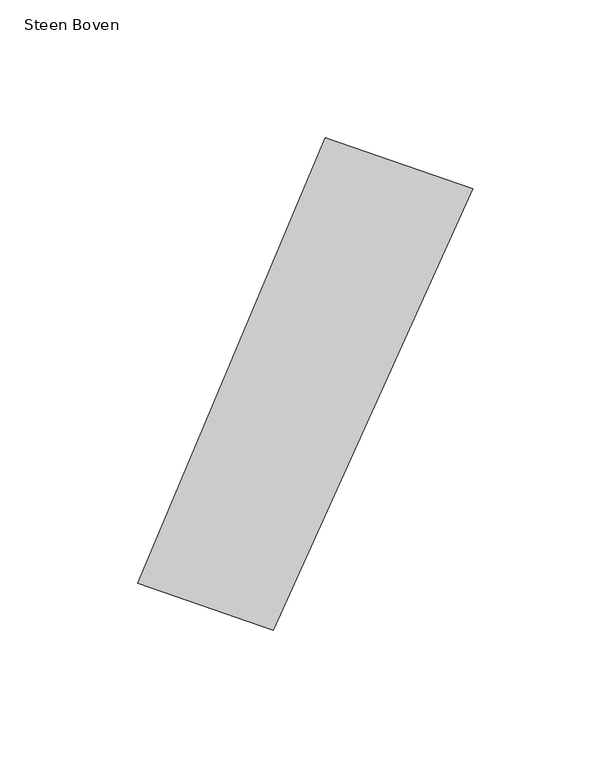
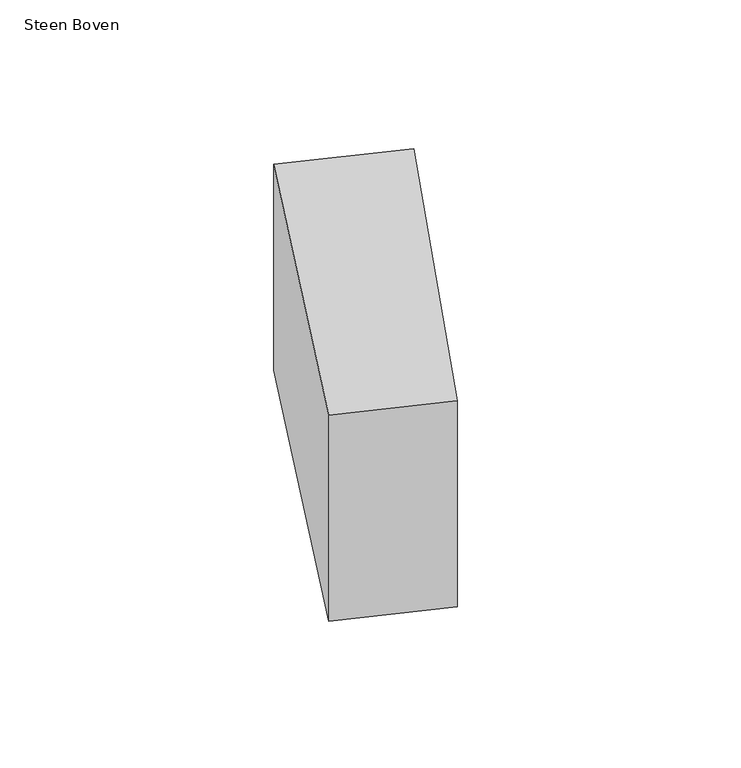
"""IFC4 building model written with IfcOpenShell, lengths in millimetres: proxy geometry, 00_GMA_steen_versie_4 : Steen Boven."""

from ifc_helpers import new_model, si_unit, origin, origin_with_axes, place, context, project, spatial, polyline, outline, extrude, source, transform, mapped, element, save


def steen_boven_7b1676e6(model_context):
    return source(origin(), model_context, "Body", "SweptSolid", [
        extrude(outline(polyline([(138.0698702, 152.5857122), (65.6416898, -7.5806935), (16.4789891, 9.3573029), (84.4906694, 171.0351119), (138.0698702, 152.5857122)])), origin_with_axes(), (0.0, 0.0, 1.0), 100.0),
    ])


if __name__ == "__main__":
    model = new_model("IFC4")
    model_context = context("Model", 3, world=origin())
    ifc_project = project(units=[si_unit("LENGTHUNIT", "METRE", prefix="MILLI")], contexts=[model_context])
    site = spatial("IfcSite", under=ifc_project)
    building = spatial("IfcBuilding", under=site)
    placement = place(None, origin())
    steen_boven_shape = steen_boven_7b1676e6(model_context)
    element("IfcBuildingElementProxy", 1, Name="00_GMA_steen_versie_4 : Steen Boven", ObjectType="00_GMA_steen_versie_4 : Steen Boven", at=placement, inside=building, context=model_context, shape_type="MappedRepresentation", body=[
        mapped(steen_boven_shape, transform((0.0, 0.0, 0.0), x_axis=(1.0, 0.0, 0.0), y_axis=(0.0, 1.0, 0.0), z_axis=(0.0, 0.0, 1.0))),
    ])
    save(model, "model.ifc")

# Revit data of these elements
# Type "00_GMA_steen_versie_4 : Steen Boven"
#   StootVoegHalfBoven [instance default] = 5 mm
#   StootVoegHalf [instance default] = 5 mm
#   StootVoegBreedteOnder = 10 mm
#   StootVoegBreedteBoven = 10 mm
#   Steendikte = 100 mm
#   LintVoegOnderHalf = 5 mm
#   LintVoegOnder = 10 mm
#   LintVoegBovenHalf = 0 mm
#   LintVoegBoven = 0 mm
#   materiaal = none
#   MateriaalVoeg = none
#   Default Elevation = 0
